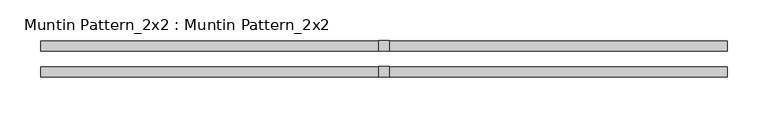
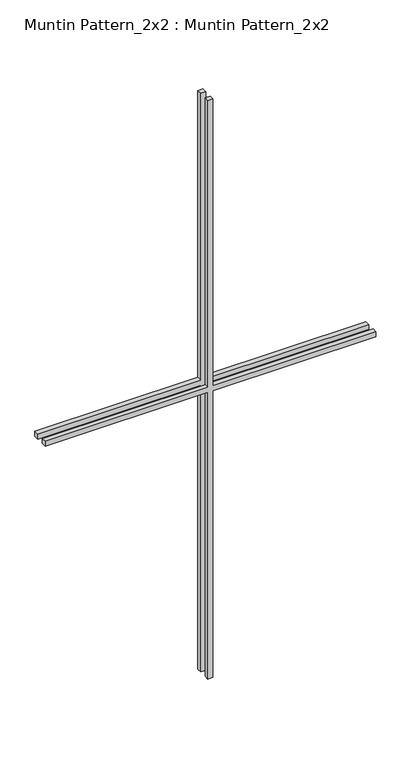
"""IFC4 building model written with IfcOpenShell, lengths in millimetres: proxy geometry, Muntin Pattern_2x2 : Muntin Pattern_2x2."""

from ifc_helpers import new_model, si_unit, frame, origin, place, context, project, spatial, polyline, outline, extrude, source, transform, mapped, element, save


def muntin_pattern_2x2_muntin_pattern_2x2_e27c8d0d(model_context):
    return source(origin(), model_context, "Body", "SweptSolid", [
        extrude(outline(polyline([(781.05, -6.35), (781.05, -419.1), (768.35, -419.1), (768.35, -6.35), (0.0, -6.35), (0.0, 6.35), (768.35, 6.35), (768.35, 419.1), (781.05, 419.1), (781.05, 6.35), (1549.4, 6.35), (1549.4, -6.35), (781.05, -6.35)])), frame((0.0, -22.225, 0.0), z_axis=(0.0, 1.0, 0.0), x_axis=(0.0, 0.0, 1.0)), (0.0, 0.0, 1.0), 12.7),
        extrude(outline(polyline([(781.05, -6.35), (781.05, -419.1), (768.35, -419.1), (768.35, -6.35), (0.0, -6.35), (0.0, 6.35), (768.35, 6.35), (768.35, 419.1), (781.05, 419.1), (781.05, 6.35), (1549.4, 6.35), (1549.4, -6.35), (781.05, -6.35)])), frame((0.0, 9.525, 0.0), z_axis=(0.0, 1.0, 0.0), x_axis=(0.0, 0.0, 1.0)), (0.0, 0.0, 1.0), 12.7),
    ])


if __name__ == "__main__":
    model = new_model("IFC4")
    model_context = context("Model", 3, world=origin())
    ifc_project = project(units=[si_unit("LENGTHUNIT", "METRE", prefix="MILLI")], contexts=[model_context])
    site = spatial("IfcSite", under=ifc_project)
    building = spatial("IfcBuilding", under=site)
    placement = place(None, origin())
    muntin_pattern_2x2_muntin_pattern_2x2_shape = muntin_pattern_2x2_muntin_pattern_2x2_e27c8d0d(model_context)
    element("IfcBuildingElementProxy", 1, Name="Muntin Pattern_2x2 : Muntin Pattern_2x2", ObjectType="Muntin Pattern_2x2 : Muntin Pattern_2x2", at=placement, inside=building, context=model_context, shape_type="MappedRepresentation", body=[
        mapped(muntin_pattern_2x2_muntin_pattern_2x2_shape, transform((0.0, 0.0, 0.0), x_axis=(1.0, 0.0, 0.0), y_axis=(0.0, 1.0, 0.0), z_axis=(0.0, 0.0, 1.0))),
    ])
    save(model, "model.ifc")

# Revit data of these elements
# Type "Muntin Pattern_2x2 : Muntin Pattern_2x2"
#   Width [instance default] = 4' - 0"
#   Thickness = 0' - 0 1/2"
#   Height [instance default] = 4' - 0"
#   Distance = 0' - 0 3/4"
#   Interior Material [instance default] = none
#   Exterior Material [instance default] = none
#   Default Elevation = 0
# Element 1 (IfcBuildingElementProxy, "Muntin Pattern_2x2 : Muntin Pattern_2x2")
#   Width = 2' - 9"
#   Height = 5' - 1"
#   Interior Material = Wood - Stained
#   Exterior Material = Clad - White
#   Materials on its faces: "Clad - White", "Wood - Stained"
# Materials
#   "Clad - White": class "Wood", colour RGB 242 242 238, transparency 0, Cost = 0
#   "Wood - Stained": class "Wood", colour RGB 224 178 126, transparency 0, Cost = 0
